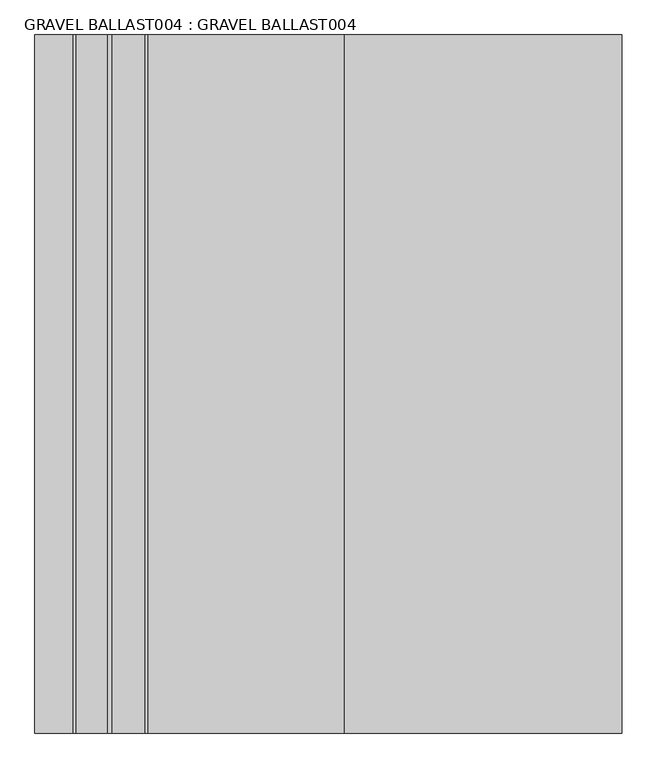
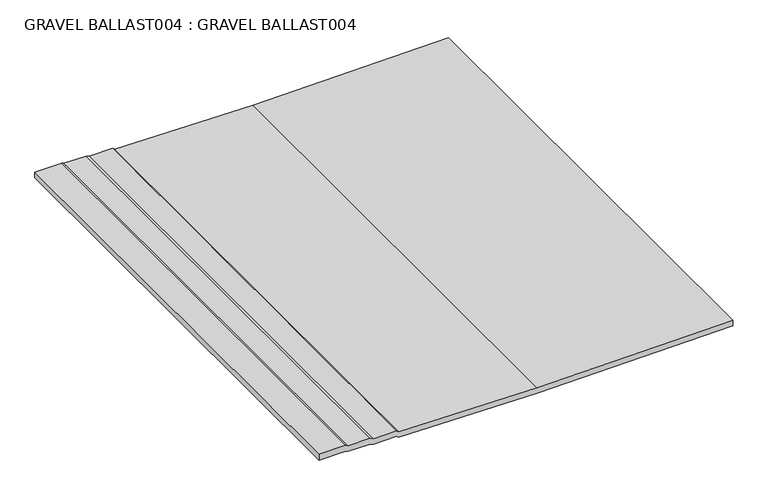
"""IFC4 building model written with IfcOpenShell, lengths in millimetres: proxy geometry, GRAVEL BALLAST004 : GRAVEL BALLAST004."""

from ifc_helpers import new_model, si_unit, frame, origin, place, context, project, spatial, polyline, outline, extrude, source, transform, mapped, element, save


def gravel_ballast004_gravel_ballast004_1e64bb1d(model_context):
    return source(origin(), model_context, "Body", "SweptSolid", [
        extrude(outline(polyline([(40274.2359465, -2672.3662777), (40269.9546965, -2663.6558285), (40269.9546965, -2573.0689144), (40264.2272344, -2560.2242751), (40265.8726651, -2466.2725277), (40258.4625089, -2457.9990902), (40250.2437589, -1894.9286556), (40261.546875, -1099.1907959), (40286.2851563, -1099.1907959), (40274.9820403, -1894.9286556), (40283.2007903, -2457.9990902), (40290.6109465, -2466.2725277), (40288.9655158, -2560.2242751), (40294.6929777, -2573.0689144), (40294.6929777, -2663.6558285), (40298.9742278, -2672.3662777), (40298.9742278, -2781.8657894), (40274.2359465, -2781.8657894), (40274.2359465, -2672.3662777)])), frame((0.0, 1000.0, 0.0), z_axis=(0.0, 1.0, 0.0), x_axis=(0.0, 0.0, 1.0)), (0.0, 0.0, 1.0), 2000.0),
    ])


if __name__ == "__main__":
    model = new_model("IFC4")
    model_context = context("Model", 3, world=origin())
    ifc_project = project(units=[si_unit("LENGTHUNIT", "METRE", prefix="MILLI")], contexts=[model_context])
    site = spatial("IfcSite", under=ifc_project)
    building = spatial("IfcBuilding", under=site)
    placement = place(None, origin())
    gravel_ballast004_gravel_ballast004_shape = gravel_ballast004_gravel_ballast004_1e64bb1d(model_context)
    element("IfcBuildingElementProxy", 1, Name="GRAVEL BALLAST004 : GRAVEL BALLAST004", ObjectType="GRAVEL BALLAST004 : GRAVEL BALLAST004", at=placement, inside=building, context=model_context, shape_type="MappedRepresentation", body=[
        mapped(gravel_ballast004_gravel_ballast004_shape, transform((0.0, 0.0, 0.0), x_axis=(1.0, 0.0, 0.0), y_axis=(0.0, 1.0, 0.0), z_axis=(0.0, 0.0, 1.0))),
    ])
    save(model, "model.ifc")

# Revit data of these elements
# Type "GRAVEL BALLAST004 : GRAVEL BALLAST004"
#   NameOverride = "GRAVEL BALLAST004"
# Element 1 (IfcBuildingElementProxy, "GRAVEL BALLAST004 : GRAVEL BALLAST004")
#   Materials on its faces: "GRAVEL BALLAST"
# Materials
#   "GRAVEL BALLAST": class "Unassigned", colour RGB 128 128 128, transparency 0, Cost = 0
